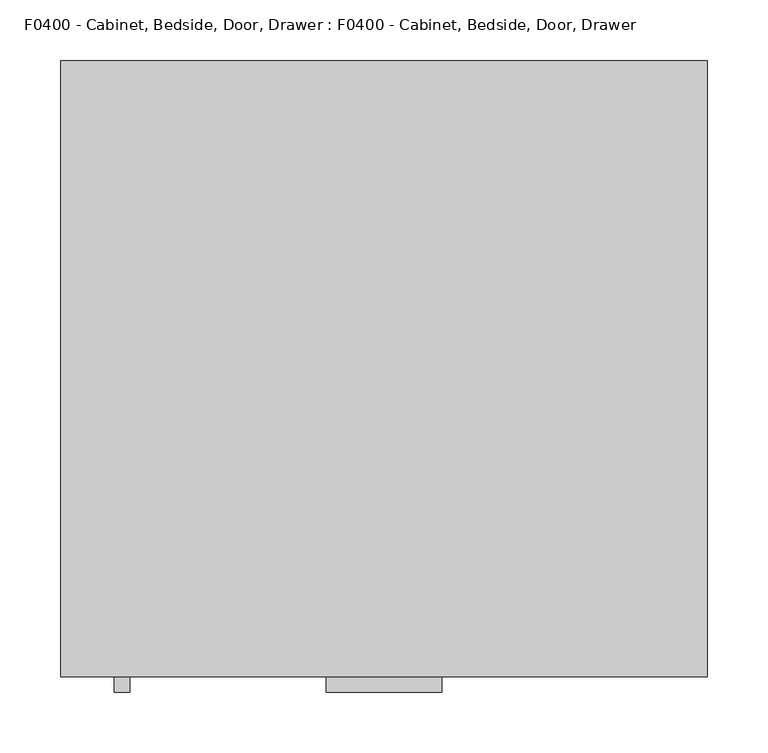
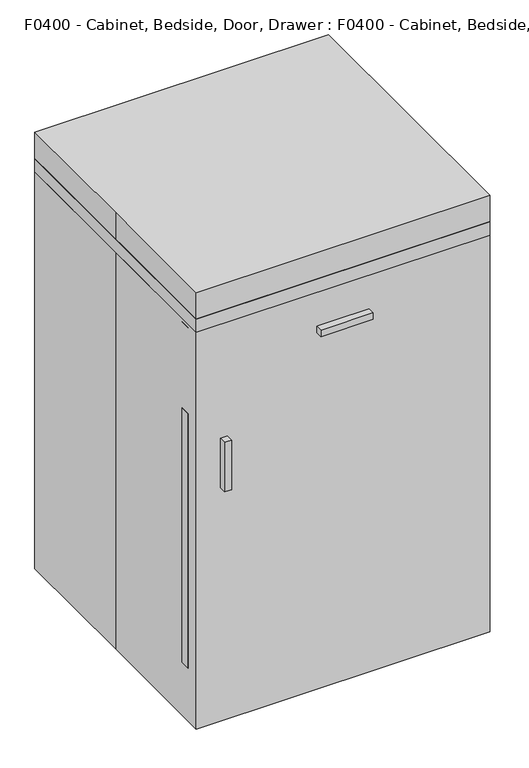
"""IFC4 building model written with IfcOpenShell, lengths in millimetres: proxy geometry, F0400 - Cabinet, Bedside, Door, Drawer : F0400 - Cabinet, Bedside, Door, Drawer."""

from ifc_helpers import new_model, si_unit, frame, origin, origin_with_axes, place, context, project, spatial, polyline, outline, extrude, source, transform, mapped, element, save


def f0400_cabinet_bedside_door_drawer_f0400_cabinet_bedside_door_b2a44ca7(model_context):
    return source(origin(), model_context, "Body", "SweptSolid", [
        extrude(outline(polyline([(0.0, -217.1558646), (0.0, -166.3558646), (101.6, -128.2558646), (101.6, -217.1558646), (0.0, -217.1558646)])), frame((0.0, -183.7187948, 0.0), z_axis=(0.0, 1.0, 0.0), x_axis=(0.0, 0.0, 1.0)), (0.0, 0.0, 1.0), 50.8),
        extrude(outline(polyline([(0.0, -217.1558646), (0.0, -166.3558646), (101.6, -128.2558646), (101.6, -217.1558646), (0.0, -217.1558646)])), frame((0.0, 165.5312052, 0.0), z_axis=(0.0, 1.0, 0.0), x_axis=(0.0, 0.0, 1.0)), (0.0, 0.0, 1.0), 50.8),
        extrude(outline(polyline([(0.0, 166.3558646), (0.0, 217.1558646), (101.6, 217.1558646), (101.6, 128.2558646), (0.0, 166.3558646)])), frame((0.0, -183.7187948, 0.0), z_axis=(0.0, 1.0, 0.0), x_axis=(0.0, 0.0, 1.0)), (0.0, 0.0, 1.0), 50.8),
        extrude(outline(polyline([(0.0, 166.3558646), (0.0, 217.1558646), (101.6, 217.1558646), (101.6, 128.2558646), (0.0, 166.3558646)])), frame((0.0, 165.5312052, 0.0), z_axis=(0.0, 1.0, 0.0), x_axis=(0.0, 0.0, 1.0)), (0.0, 0.0, 1.0), 50.8),
        extrude(outline(polyline([(247.65, 234.95), (247.65, -209.55), (-247.65, -209.55), (-247.65, 234.95), (247.65, 234.95)])), frame((0.0, 0.0, 101.6), z_axis=(0.0, 0.0, 1.0), x_axis=(1.0, 0.0, 0.0)), (0.0, 0.0, 1.0), 19.05),
        extrude(outline(polyline([(-266.7159299, 447.6560937), (-266.7159299, 542.9060937), (-228.6159299, 542.9060937), (-228.6159299, 530.2220236), (-254.0318599, 530.2220236), (-254.0318599, 460.3401637), (-228.6159299, 460.3401637), (-228.6159299, 447.6560937), (-266.7159299, 447.6560937)])), frame((-222.5434712, 0.0, 0.0), z_axis=(1.0, 0.0, 0.0), x_axis=(0.0, 1.0, 0.0)), (0.0, 0.0, 1.0), 12.7),
        extrude(outline(polyline([(-47.625, -266.7159299), (-47.625, -228.6159299), (-34.9409299, -228.6159299), (-34.9409299, -254.0318599), (34.9409299, -254.0318599), (34.9409299, -228.6159299), (47.625, -228.6159299), (47.625, -266.7159299), (-47.625, -266.7159299)])), frame((0.0, 0.0, 684.1962383), z_axis=(0.0, 0.0, 1.0), x_axis=(1.0, 0.0, 0.0)), (0.0, 0.0, 1.0), 12.7),
        extrude(outline(polyline([(266.7, 254.0), (266.7, -254.0), (-266.7, -254.0), (-266.7, 254.0), (266.7, 254.0)])), frame((0.0, 0.0, 762.0), z_axis=(0.0, 0.0, 1.0), x_axis=(1.0, 0.0, 0.0)), (0.0, 0.0, 1.0), 25.4),
        extrude(outline(polyline([(266.7, -228.6), (-266.7, -228.6), (-266.7, -209.55), (266.7, -209.55), (266.7, -228.6)])), frame((0.0, 0.0, 101.6), z_axis=(0.0, 0.0, 1.0), x_axis=(1.0, 0.0, 0.0)), (0.0, 0.0, 1.0), 488.95),
        extrude(outline(polyline([(-266.7, 254.0), (266.7, 254.0), (266.7, -254.0), (-266.7, -254.0), (-266.7, 0.0), (-266.7, 254.0)])), origin_with_axes(), (0.0, 0.0, 1.0), 838.2),
        extrude(outline(polyline([(266.7, -228.6), (-266.7, -228.6), (-266.7, -209.55), (266.7, -209.55), (266.7, -228.6)])), frame((0.0, 0.0, 596.9), z_axis=(0.0, 0.0, 1.0), x_axis=(1.0, 0.0, 0.0)), (0.0, 0.0, 1.0), 158.7174767),
        extrude(outline(polyline([(247.65, 234.95), (-247.65, 234.95), (-247.65, 254.0), (247.65, 254.0), (247.65, 234.95)])), frame((0.0, 0.0, 101.6), z_axis=(0.0, 0.0, 1.0), x_axis=(1.0, 0.0, 0.0)), (0.0, 0.0, 1.0), 660.4),
        extrude(outline(polyline([(-266.7, -228.6), (-266.7, 254.0), (-247.65, 254.0), (-247.65, -228.6), (-266.7, -228.6)])), frame((0.0, 0.0, 101.6), z_axis=(0.0, 0.0, 1.0), x_axis=(1.0, 0.0, 0.0)), (0.0, 0.0, 1.0), 660.4),
        extrude(outline(polyline([(247.65, -228.6), (247.65, 254.0), (266.7, 254.0), (266.7, -228.6), (247.65, -228.6)])), frame((0.0, 0.0, 101.6), z_axis=(0.0, 0.0, 1.0), x_axis=(1.0, 0.0, 0.0)), (0.0, 0.0, 1.0), 660.4),
    ])


if __name__ == "__main__":
    model = new_model("IFC4")
    model_context = context("Model", 3, world=origin())
    ifc_project = project(units=[si_unit("LENGTHUNIT", "METRE", prefix="MILLI")], contexts=[model_context])
    site = spatial("IfcSite", under=ifc_project)
    building = spatial("IfcBuilding", under=site)
    placement = place(None, origin())
    f0400_cabinet_bedside_door_drawer_f0400_cabinet_bedside_door_shape = f0400_cabinet_bedside_door_drawer_f0400_cabinet_bedside_door_b2a44ca7(model_context)
    element("IfcBuildingElementProxy", 1, Name="F0400 - Cabinet, Bedside, Door, Drawer : F0400 - Cabinet, Bedside, Door, Drawer", ObjectType="F0400 - Cabinet, Bedside, Door, Drawer : F0400 - Cabinet, Bedside, Door, Drawer", at=placement, inside=building, context=model_context, shape_type="MappedRepresentation", body=[
        mapped(f0400_cabinet_bedside_door_drawer_f0400_cabinet_bedside_door_shape, transform((0.0, 0.0, 0.0), x_axis=(1.0, 0.0, 0.0), y_axis=(0.0, 1.0, 0.0), z_axis=(0.0, 0.0, 1.0))),
    ])
    save(model, "model.ifc")

# Revit data of these elements
# Type "F0400 - Cabinet, Bedside, Door, Drawer : F0400 - Cabinet, Bedside, Door, Drawer"
#   Watts2 = "0"
#   Watts1 = "0"
#   Unit_Issue = "EA"
#   UTIL_6_Misc = "-"
#   UTIL_5_NonMedGas = "-"
#   UTIL_4_MiscGas = "-"
#   UTIL_3_MedGas = "-"
#   UTIL_2_Elec = "-"
#   UTIL_1_WaterDrain = "-"
#   Nomenclature = "Cabinet, Bedside, Door, Drawer"
#   NSN = "6530"
#   Location [instance default] = ""
#   JSN = "F0400"
#   Fund_Source_VA = "-"
#   Fund_Source_Navy = "-"
#   Fund_Source_Army = "-"
#   Fund_Source_AF = "-"
#   ELEC_Volts2 = "0"
#   ELEC_Volts1 = "0"
#   ELEC_Phase2 = "0"
#   ELEC_Phase1 = "0"
#   ELEC_HertzSwitch = "0"
#   ELEC_HertzDependent = "0"
#   ELEC_Hertz = "0"
#   ELEC_Amps2 = "0"
#   ELEC_Amps1 = "0"
#   DetailDescription = "Bedside cabinet for storage of both the patient's personal items and small patient support items. Approximately 31\" high X 21\" wide X 19\" deep with one (1) drawer and one (1) closed storage closet. Drawer is removable so interior can be sanitized. May come in a 3 drawer version."
#   CAT_VA = "A"
#   CAT_Navy = "A"
#   CAT_IHS = "-"
#   CAT_Army = "A"
#   CAT_AF = "A"
#   BTUperhour = "0"
#   Weight_IP = 80
#   DIM_Width_IP = 1' - 9"
#   DIM_Height_IP = 2' - 9"
#   DIM_Depth_IP = 1' - 8"
#   Top Panel Material = none
#   Toe Panel Material = none
#   Side Panel Material = none
#   Shelf Panel Material = none
#   Drawer Front Material = none
#   Door Panel Material = none
#   Back Panel Material = none
#   Assembly Code = ""
# Element 1 (IfcBuildingElementProxy, "F0400 - Cabinet, Bedside, Door, Drawer : F0400 - Cabinet, Bedside, Door, Drawer")
#   Location = "BRMS1"
#   Materials on its faces: "Default metal", "EquipSpace"
# Materials
#   "Default metal": class "Unassigned", colour RGB 204 204 204, transparency 0
#   "EquipSpace": class "Unassigned", colour RGB 221 217 195, transparency 0.5
